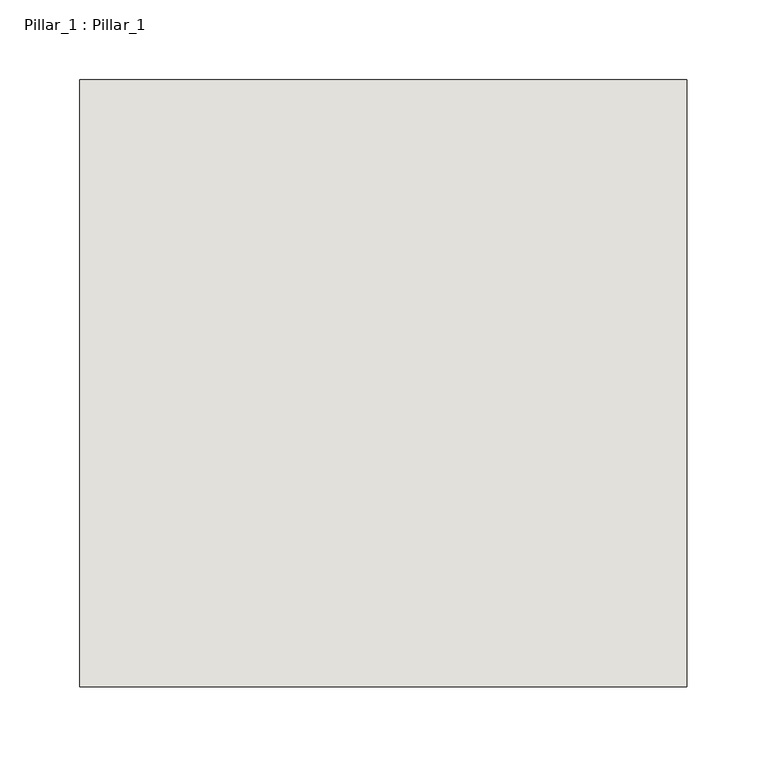
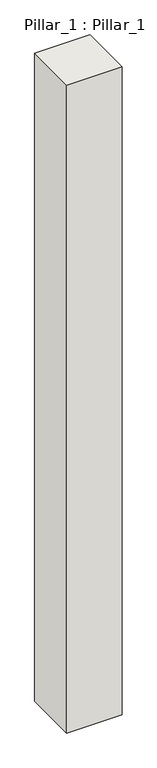
"""IFC4 building model written with IfcOpenShell, lengths in millimetres: wall geometry, Pillar_1 : Pillar_1."""

from ifc_helpers import new_model, si_unit, origin, origin_with_axes, place, context, project, spatial, polyline, outline, extrude, source, transform, mapped, element, save


def pillar_1_pillar_1_f30ecb4e(model_context):
    return source(origin(), model_context, "Body", "SweptSolid", [
        extrude(outline(polyline([(240.0, 0.0), (-140.0, 0.0), (-140.0, 380.0), (240.0, 380.0), (240.0, 0.0)])), origin_with_axes(), (0.0, 0.0, 1.0), 4700.0),
    ])


if __name__ == "__main__":
    model = new_model("IFC4")
    model_context = context("Model", 3, world=origin())
    ifc_project = project(units=[si_unit("LENGTHUNIT", "METRE", prefix="MILLI")], contexts=[model_context])
    site = spatial("IfcSite", under=ifc_project)
    building = spatial("IfcBuilding", under=site)
    placement = place(None, origin())
    pillar_1_pillar_1_shape = pillar_1_pillar_1_f30ecb4e(model_context)
    element("IfcWall", 1, ObjectType="Pillar_1 : Pillar_1", at=placement, inside=building, context=model_context, shape_type="MappedRepresentation", body=[
        mapped(pillar_1_pillar_1_shape, transform((0.0, 0.0, 0.0), x_axis=(1.0, 0.0, 0.0), y_axis=(0.0, 1.0, 0.0), z_axis=(0.0, 0.0, 1.0))),
    ])
    save(model, "model.ifc")

# Revit data of these elements
# Type "Pillar_1 : Pillar_1"
#   NameOverride = "Pillar_1"
# Element 1 (IfcWall, "Pillar_1 : Pillar_1")
#   Materials on its faces: "IfcSurfaceStyle #33"
# Materials
#   "IfcSurfaceStyle #33": class "Unassigned", colour RGB 214 214 214, transparency 0
